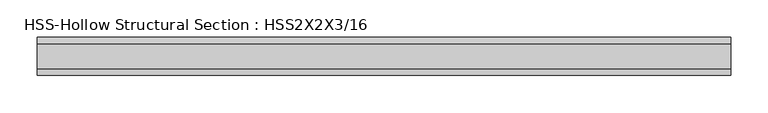
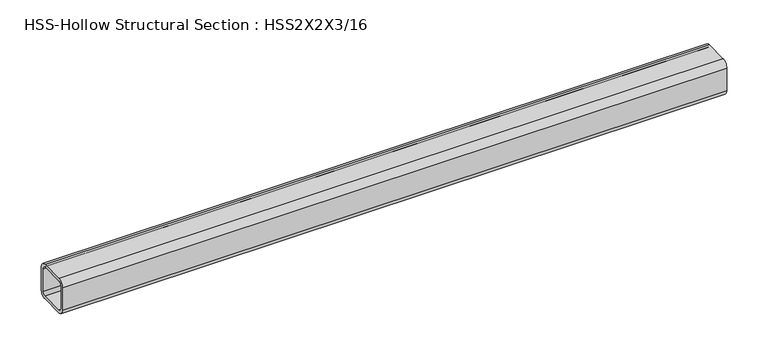
"""IFC4 building model written with IfcOpenShell, lengths in millimetres: beam geometry, HSS-Hollow Structural Section : HSS2X2X3/16."""

from ifc_helpers import new_model, si_unit, point, frame, frame_2d, origin, place, context, project, spatial, polyline, circle_curve, trimmed, segment, composite_curve, outline, extrude, source, transform, mapped, element, save


def hss_hollow_structural_section_hss2x2x3_16_b6e2ff5b(model_context):
    return source(origin(), model_context, "Body", "SweptSolid", [
        extrude(outline(composite_curve([segment(polyline([(25.4, 16.5608), (25.4, -16.5608)]), True, "CONTINUOUS"), segment(trimmed(circle_curve(frame_2d((16.5608, -16.5608)), 8.8392), [point((25.4, -16.5608))], [point((16.5608, -25.4))], False, "CARTESIAN"), True, "CONTINUOUS"), segment(polyline([(16.5608, -25.4), (-16.5608, -25.4)]), True, "CONTINUOUS"), segment(trimmed(circle_curve(frame_2d((-16.5608, -16.5608)), 8.8392), [point((-16.5608, -25.4))], [point((-25.4, -16.5608))], False, "CARTESIAN"), True, "CONTINUOUS"), segment(polyline([(-25.4, -16.5608), (-25.4, 16.5608)]), True, "CONTINUOUS"), segment(trimmed(circle_curve(frame_2d((-16.5608, 16.5608)), 8.8392), [point((-25.4, 16.5608))], [point((-16.5608, 25.4))], False, "CARTESIAN"), True, "CONTINUOUS"), segment(polyline([(-16.5608, 25.4), (16.5608, 25.4)]), True, "CONTINUOUS"), segment(trimmed(circle_curve(frame_2d((16.5608, 16.5608)), 8.8392), [point((16.5608, 25.4))], [point((25.4, 16.5608))], False, "CARTESIAN"), True, "CONTINUOUS")], self_intersect=False), holes=[composite_curve([segment(trimmed(circle_curve(frame_2d((-16.5608, 16.5608)), 4.4196), [point((-16.5608, 20.9804))], [point((-20.9804, 16.5608))], True, "CARTESIAN"), True, "CONTINUOUS"), segment(polyline([(-20.9804, 16.5608), (-20.9804, -16.5608)]), True, "CONTINUOUS"), segment(trimmed(circle_curve(frame_2d((-16.5608, -16.5608)), 4.4196), [point((-20.9804, -16.5608))], [point((-16.5608, -20.9804))], True, "CARTESIAN"), True, "CONTINUOUS"), segment(polyline([(-16.5608, -20.9804), (16.5608, -20.9804)]), True, "CONTINUOUS"), segment(trimmed(circle_curve(frame_2d((16.5608, -16.5608)), 4.4196), [point((16.5608, -20.9804))], [point((20.9804, -16.5608))], True, "CARTESIAN"), True, "CONTINUOUS"), segment(polyline([(20.9804, -16.5608), (20.9804, 16.5608)]), True, "CONTINUOUS"), segment(trimmed(circle_curve(frame_2d((16.5608, 16.5608)), 4.4196), [point((20.9804, 16.5608))], [point((16.5608, 20.9804))], True, "CARTESIAN"), True, "CONTINUOUS"), segment(polyline([(16.5608, 20.9804), (-16.5608, 20.9804)]), True, "CONTINUOUS")], self_intersect=False)]), frame((8535.19375, 0.0, 0.0), z_axis=(1.0, 0.0, 0.0), x_axis=(0.0, 1.0, 0.0)), (0.0, 0.0, 1.0), 927.1),
    ])


if __name__ == "__main__":
    model = new_model("IFC4")
    model_context = context("Model", 3, world=origin())
    ifc_project = project(units=[si_unit("LENGTHUNIT", "METRE", prefix="MILLI")], contexts=[model_context])
    site = spatial("IfcSite", under=ifc_project)
    building = spatial("IfcBuilding", under=site)
    placement = place(None, origin())
    hss_hollow_structural_section_hss2x2x3_16_shape = hss_hollow_structural_section_hss2x2x3_16_b6e2ff5b(model_context)
    element("IfcBeam", 1, ObjectType="HSS-Hollow Structural Section : HSS2X2X3/16", at=placement, inside=building, context=model_context, shape_type="MappedRepresentation", body=[
        mapped(hss_hollow_structural_section_hss2x2x3_16_shape, transform((0.0, 0.0, 0.0), x_axis=(1.0, 0.0, 0.0), y_axis=(0.0, 1.0, 0.0), z_axis=(0.0, 0.0, 1.0))),
    ])
    save(model, "model.ifc")

# Revit data of these elements
# Type "HSS-Hollow Structural Section : HSS2X2X3/16"
#   Keynote = "M05121300.04"
#   Assembly Code = "B10"
#   Shape = "Square"
#   W = 4.3
#   Ht = 0' - 2"
#   Length [instance default] = 5' - 0"
#   b = 0' - 2"
#   kr = 0' - 0.348"
#   t = 0' - 0.174"
#   A = 0.00826389 SF
#   Structural Material [instance default] = Steel ASTM A500, Grade B, Rectangular and Square
# Element 1 (IfcBeam, "HSS-Hollow Structural Section : HSS2X2X3/16")
#   Materials on its faces: "Steel ASTM A500, Grade B, Rectangular and Square"
# Materials
#   "Steel ASTM A500, Grade B, Rectangular and Square": class "Metal", colour RGB 199 199 199, transparency 0, Description = "Carbon steel", Cost = 0
